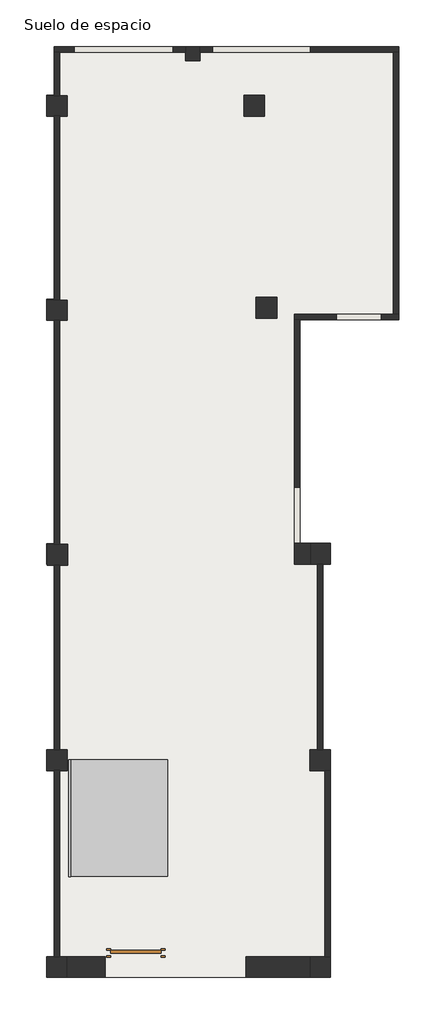
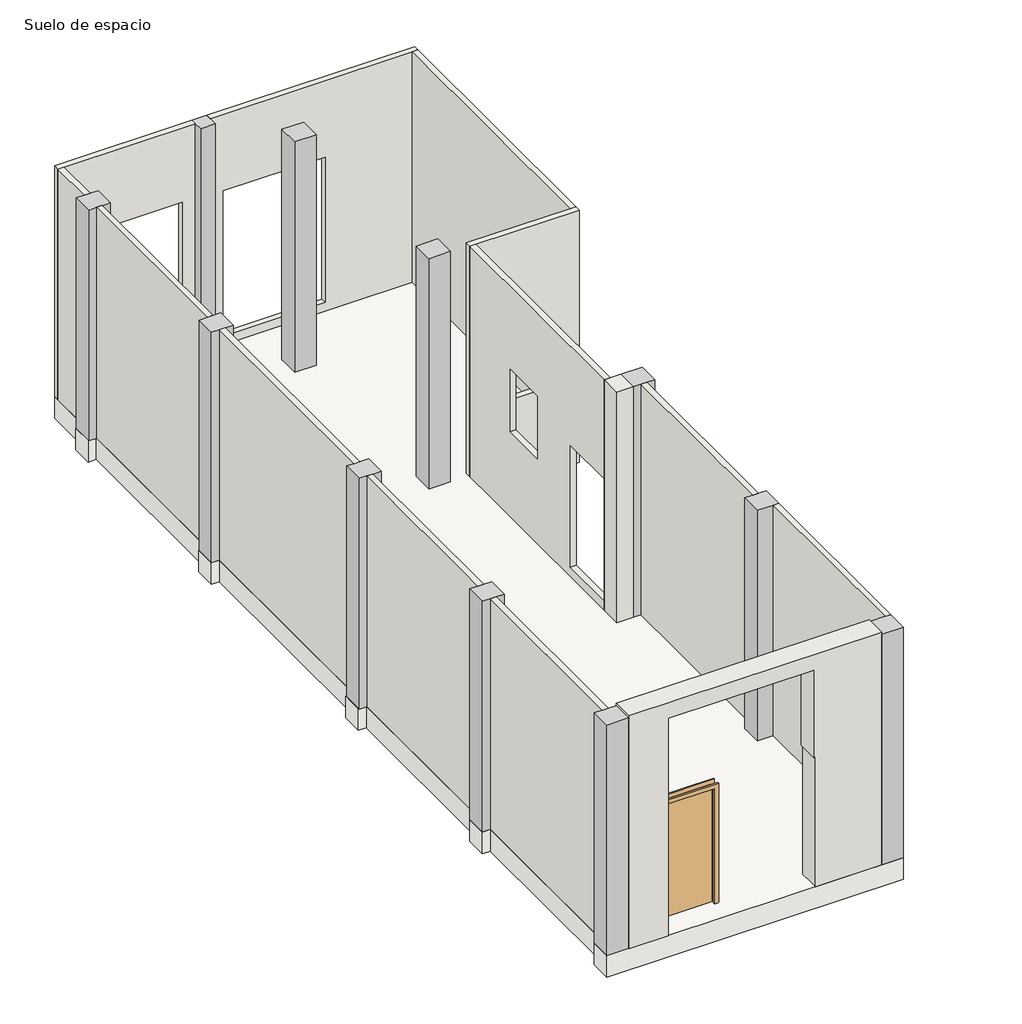
# One storey: 14 walls, 11 columns, 1 door, 1 railing, 1 ramp, 1 slab.
# Revit data of these elements (continued)
# Element 14 (IfcRamp, "Ramp 1") (continued)
#   Width = 179.0 cm
#   built-in parameter 1007276 = 1
#   built-in parameter 1007274 = 1
#   built-in parameter 1007273 = 1
#   built-in parameter 1007271 = 1
#   Phase Created = New Construction
# Element 15 (IfcSlab, "Generic Floor - 400mm")
#   Height Offset From Level = 0.0 cm
#   Phase Created = New Construction
#   Materials on its faces: "Default Roof"
# Elements 16, 17, 18, 19, 20, 21, 22, 23, 24, 25, 26, 27 (IfcWall, "Generic - 100mm Masonry")
#   Top Offset = 0.0 cm
#   Base Offset = 0.0 cm
#   wall height = 426.0 cm
#   Phase Created = Existing
#   Base Constraint = Suelo de espacio
#   Top Constraint = Techo de espacio
#   Materials on its faces: "Concrete, Cast-in-Place gray"
# Element 28 (IfcWall, "Generic - 380mm Masonry")
#   Top Offset = 0.0 cm
#   Base Offset = 0.0 cm
#   wall height = 426.0 cm
#   Phase Created = Existing
#   Base Constraint = Suelo de espacio
#   Top Constraint = Techo de espacio
#   Materials on its faces: "Concrete, Cast-in-Place gray"
# Element 29 (IfcWall, "Generic - 380mm Masonry")
#   Top Offset = 0.0 cm
#   Base Offset = 0.0 cm
#   Unconnected Height = 430.0 cm
#   wall height = 430.0 cm
#   Phase Created = Existing
#   Base Constraint = Suelo de espacio
#   Materials on its faces: "Concrete, Cast-in-Place gray"
# Materials
#   "Door - Panel": class "Wood", colour RGB 114 82 51, transparency 0
#   "Door - Frame": class "Miscellaneous", colour RGB 153 76 43, transparency 0
#   "Concrete, Cast-in-Place gray": class "Concrete", colour RGB 115 116 108, transparency 0, Description = "Cast-in-place concrete", Cost = 0
#   "Default Roof": class "Miscellaneous", colour RGB 80 80 80, transparency 0
